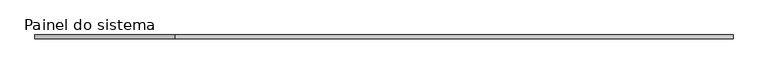
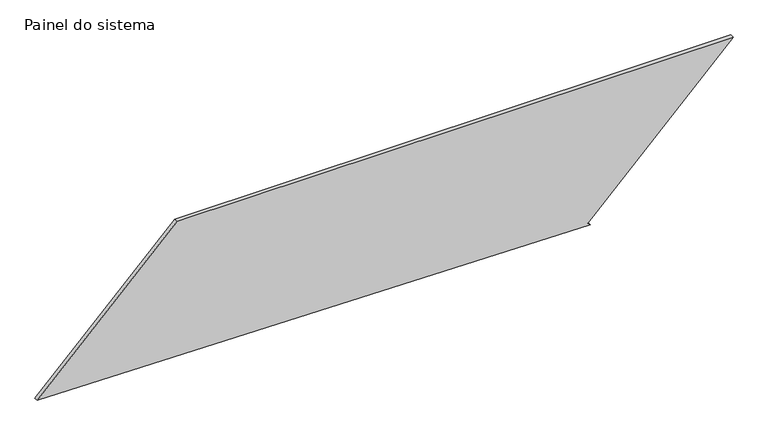
"""IFC4 building model written with IfcOpenShell, lengths in millimetres: plate geometry, Painel do sistema : Envidraçado."""

from ifc_helpers import new_model, si_unit, frame, origin, place, context, project, spatial, polyline, outline, extrude, source, transform, mapped, element, save


def painel_do_sistema_c99de997(model_context):
    return source(origin(), model_context, "Body", "SweptSolid", [
        extrude(outline(polyline([(0.0, 1328.8466464), (17.655268, 1311.1466038), (961.1998316, 2252.3043449), (961.1998316, -1346.0329596), (52.6300974, -2252.3043449), (0.0, 1328.8466464)])), frame((0.0, 24.5, 0.0), z_axis=(0.0, 1.0, 0.0), x_axis=(0.0, 0.0, 1.0)), (0.0, 0.0, 1.0), 25.0),
    ])


if __name__ == "__main__":
    model = new_model("IFC4")
    model_context = context("Model", 3, world=origin())
    ifc_project = project(units=[si_unit("LENGTHUNIT", "METRE", prefix="MILLI")], contexts=[model_context])
    site = spatial("IfcSite", under=ifc_project)
    building = spatial("IfcBuilding", under=site)
    placement = place(None, origin())
    painel_do_sistema_shape = painel_do_sistema_c99de997(model_context)
    element("IfcPlate", 1, ObjectType="Painel do sistema : Envidraçado", at=placement, inside=building, context=model_context, shape_type="MappedRepresentation", body=[
        mapped(painel_do_sistema_shape, transform((0.0, 0.0, 0.0), x_axis=(1.0, 0.0, 0.0), y_axis=(0.0, 1.0, 0.0), z_axis=(0.0, 0.0, 1.0))),
    ])
    save(model, "model.ifc")

# Revit data of these elements
# Type "Painel do sistema : Envidraçado"
#   Construction Type Id = "GSP4R"
#   Analytic Construction = "Vidraça única Pilkington 1/8 pol"
#   Visual Light Transmittance = 0.9
#   Solar Heat Gain Coefficient = 0.86
#   Heat Transfer Coefficient (U) = 6.7069 W/(m²·K)
# Element 1 (IfcPlate, "Painel do sistema : Envidraçado")
#   Materials on its faces: "Vidro"
# Materials
#   "Vidro": class "Vidro", colour RGB 0 128 192, transparency 0.9, Description = "Vidro de sílica", Cost = 0
